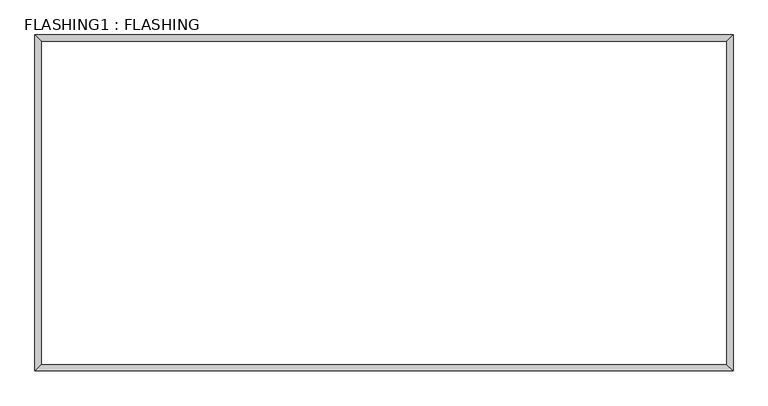
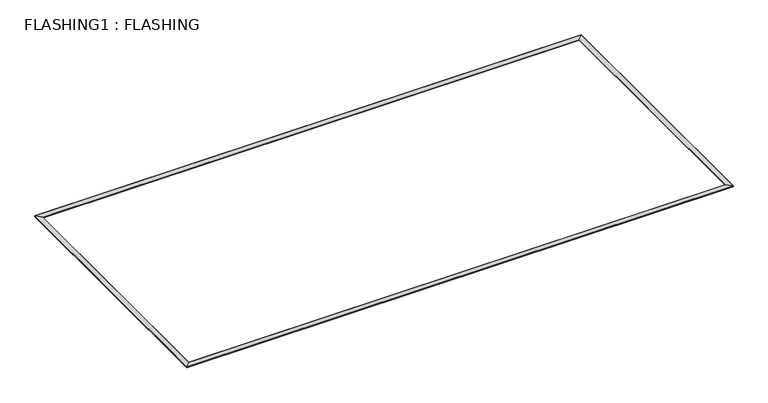
"""IFC4 building model written with IfcOpenShell, lengths in millimetres: proxy geometry, FLASHING1 : FLASHING."""

import ifcopenshell
import ifcopenshell.guid

model = None  # the IFC model being written
_history = None  # IfcOwnerHistory: only IFC2X3 demands one
_inside = {}  # id of a spatial element -> (the spatial element, [elements in it])
_under = {}  # id of a project, library or spatial element -> (it, [spatial elements below it])
_declared = {}  # id of a project -> (the project, [libraries it declares])
_typed = {}  # id of a type object -> (the type object, [elements of that type])
_made_of = {}  # id of a material, layer set ... -> (it, [elements and type objects made of it])


def new_model(schema):
    """Start an empty IFC model of exactly this schema.

    Asked for "IFC4X3", IfcOpenShell would pick the latest addendum, in which some entities
    have other attributes; the version numbers below select the first issue.
    IFC2X3 requires an IfcOwnerHistory on every rooted entity: one is made here for all.
    """
    global model, _history
    if schema == "IFC4X3":
        model = ifcopenshell.file(schema_version=(4, 3, 0, 0))
    else:
        model = ifcopenshell.file(schema=schema)
    _inside.clear()
    _under.clear()
    _declared.clear()
    _typed.clear()
    _made_of.clear()
    _history = None
    if model.schema == "IFC2X3":
        org = make("IfcOrganization", Name="unknown")
        user = make(
            "IfcPersonAndOrganization",
            ThePerson=make("IfcPerson", FamilyName="unknown"),
            TheOrganization=org,
        )
        app = make(
            "IfcApplication",
            ApplicationDeveloper=org,
            Version="unknown",
            ApplicationFullName="unknown",
            ApplicationIdentifier="unknown",
        )
        _history = make(
            "IfcOwnerHistory",
            OwningUser=user,
            OwningApplication=app,
            ChangeAction="ADDED",
            CreationDate=0,
        )
    return model


def make(cls, **values):
    """One entity of the class cls with the attributes given. An attribute that is None is left unset."""
    return model.create_entity(
        cls, **{name: value for name, value in values.items() if value is not None}
    )


def rooted(cls, **values):
    """An entity with a GlobalId (a new one), such as an element, a storey or a relation."""
    return make(cls, GlobalId=ifcopenshell.guid.new(), OwnerHistory=_history, **values)


def si_unit(unit_type, name, prefix=None):
    """IfcSIUnit, for example si_unit("LENGTHUNIT", "METRE", prefix="MILLI")."""
    return make("IfcSIUnit", UnitType=unit_type, Prefix=prefix, Name=name)


def assignment(units):
    """IfcUnitAssignment: the units of a project."""
    return None if units is None else make("IfcUnitAssignment", Units=units)


def point(xyz):
    """IfcCartesianPoint."""
    return None if xyz is None else make("IfcCartesianPoint", Coordinates=xyz)


def direction(xyz):
    """IfcDirection."""
    return None if xyz is None else make("IfcDirection", DirectionRatios=xyz)


def frame(location, z_axis=None, x_axis=None):
    """IfcAxis2Placement3D, a coordinate frame: its origin and axes. An axis left out is left unset."""
    return make(
        "IfcAxis2Placement3D",
        Location=point(location),
        Axis=direction(z_axis),
        RefDirection=direction(x_axis),
    )


def origin():
    """The frame at (0, 0, 0) with its axes left unset."""
    return frame((0.0, 0.0, 0.0))


def place(relative_to, where):
    """IfcLocalPlacement: puts the frame where relative to a parent placement (None: the world)."""
    return make(
        "IfcLocalPlacement", PlacementRelTo=relative_to, RelativePlacement=where
    )


def context(
    kind, dimensions, precision=None, world=None, true_north=None, identifier=None
):
    """IfcGeometricRepresentationContext, for example the 3D "Model" context."""
    return make(
        "IfcGeometricRepresentationContext",
        ContextIdentifier=identifier,
        ContextType=kind,
        CoordinateSpaceDimension=dimensions,
        Precision=precision,
        WorldCoordinateSystem=world,
        TrueNorth=true_north,
    )


def project(units=None, contexts=None):
    """IfcProject with its units and contexts."""
    return rooted(
        "IfcProject",
        Name="project",
        RepresentationContexts=contexts,
        UnitsInContext=assignment(units),
    )


def spatial(cls, under=None, at=None, **own):
    """A site, building, storey or space (cls), placed at a placement, below another one or the project."""
    s = rooted(cls, ObjectPlacement=at, **own)
    if under is not None:
        _under.setdefault(under.id(), (under, []))[1].append(s)
    return s


def faces_of(points, faces, orient=None, outer=None):
    """IfcFace entities. A face is a list of loops; a loop is a list of indices into points, from 0.

    orient and outer hold one flag for each loop. By default every Orientation is true, the
    first loop of a face is its IfcFaceOuterBound and the others are IfcFaceBound.
    """
    made = []
    for i, loops in enumerate(faces):
        bounds = []
        for j, loop in enumerate(loops):
            is_outer = j == 0 if outer is None else outer[i][j]
            bounds.append(
                make(
                    "IfcFaceOuterBound" if is_outer else "IfcFaceBound",
                    Bound=make("IfcPolyLoop", Polygon=[points[k] for k in loop]),
                    Orientation=True if orient is None else orient[i][j],
                )
            )
        made.append(make("IfcFace", Bounds=bounds))
    return made


def faceted_brep(points, faces, orient=None, outer=None, voids=None):
    """IfcFacetedBrep: a solid bounded by flat faces; with voids (closed shells), ...WithVoids."""
    shared = [point(p) for p in points]
    hull = make("IfcClosedShell", CfsFaces=faces_of(shared, faces, orient, outer))
    if voids is None:
        return make("IfcFacetedBrep", Outer=hull)
    return make(
        "IfcFacetedBrepWithVoids",
        Outer=hull,
        Voids=[
            make(cls, CfsFaces=faces_of(shared, fs, o, b)) for cls, fs, o, b in voids
        ],
    )


def shape(context_of_items, identifier, shape_type, items):
    """IfcShapeRepresentation: the items that make up one representation, for example the "Body"."""
    return make(
        "IfcShapeRepresentation",
        ContextOfItems=context_of_items,
        RepresentationIdentifier=identifier,
        RepresentationType=shape_type,
        Items=items,
    )


def source(mapping_origin, context_of_items, identifier, shape_type, items):
    """IfcRepresentationMap: a shape defined once, which mapped items show again and again."""
    return make(
        "IfcRepresentationMap",
        MappingOrigin=mapping_origin,
        MappedRepresentation=shape(context_of_items, identifier, shape_type, items),
    )


def transform(
    local_origin,
    x_axis=None,
    y_axis=None,
    z_axis=None,
    scale=None,
    scale2=None,
    scale3=None,
    uniform=True,
):
    """IfcCartesianTransformationOperator3D, or its non-uniform kind. x_axis, y_axis, z_axis: its Axis1, 2, 3."""
    if uniform:
        return make(
            "IfcCartesianTransformationOperator3D",
            Axis1=direction(x_axis),
            Axis2=direction(y_axis),
            LocalOrigin=point(local_origin),
            Scale=scale,
            Axis3=direction(z_axis),
        )
    return make(
        "IfcCartesianTransformationOperator3DnonUniform",
        Axis1=direction(x_axis),
        Axis2=direction(y_axis),
        LocalOrigin=point(local_origin),
        Scale=scale,
        Axis3=direction(z_axis),
        Scale2=scale2,
        Scale3=scale3,
    )


def mapped(mapping_source, mapping_target):
    """IfcMappedItem: shows the shape of a source again, moved by a transform."""
    return make(
        "IfcMappedItem", MappingSource=mapping_source, MappingTarget=mapping_target
    )


def made_of(thing, what):
    """Note that an element or type object is made of a material, layer set ...; save() writes the relation."""
    if what is not None:
        _made_of.setdefault(what.id(), (what, []))[1].append(thing)
    return thing


def element(
    cls,
    number,
    at=None,
    inside=None,
    cuts=None,
    type_object=None,
    material=None,
    context=None,
    identifier="Body",
    shape_type=None,
    held_by="IfcProductDefinitionShape",
    body=None,
    shapes=None,
    **own,
):
    """One element of the class cls, such as IfcWall. Its Tag is "e" and its number.

    at: its placement. inside: the storey or other place that contains it. cuts: it is an
    opening in that element (IfcRelVoidsElement). A single representation is given by context,
    identifier, shape_type and body (its items); several are given by shapes. held_by: the class
    of the entity that holds the representations. save() writes the other relations.
    """
    e = rooted(cls, Tag="e%d" % number, ObjectPlacement=at, **own)
    if body is not None:
        shapes = [shape(context, identifier, shape_type, body)]
    if shapes is not None:
        e.Representation = make(held_by, Representations=shapes)
    if inside is not None:
        _inside.setdefault(inside.id(), (inside, []))[1].append(e)
    if cuts is not None:
        rooted(
            "IfcRelVoidsElement", RelatingBuildingElement=cuts, RelatedOpeningElement=e
        )
    if type_object is not None:
        _typed.setdefault(type_object.id(), (type_object, []))[1].append(e)
    return made_of(e, material)


def aggregate(whole, parts):
    """IfcRelAggregates: a whole, such as a stair, and the parts it consists of."""
    return rooted("IfcRelAggregates", RelatingObject=whole, RelatedObjects=parts)


def save(model, path):
    """Write the relations noted so far, then the file.

    IfcRelAggregates (storeys below a building ...), IfcRelContainedInSpatialStructure (elements
    in a storey), IfcRelDefinesByType, IfcRelAssociatesMaterial and IfcRelDeclares: one each for
    every whole, place, type object, material and project.
    """
    for whole, parts in _under.values():
        aggregate(whole, parts)
    for where, things in _inside.values():
        rooted(
            "IfcRelContainedInSpatialStructure",
            RelatedElements=things,
            RelatingStructure=where,
        )
    for kind, things in _typed.values():
        rooted("IfcRelDefinesByType", RelatedObjects=things, RelatingType=kind)
    for what, things in _made_of.values():
        rooted("IfcRelAssociatesMaterial", RelatedObjects=things, RelatingMaterial=what)
    for by, libraries in _declared.values():
        rooted("IfcRelDeclares", RelatingContext=by, RelatedDefinitions=libraries)
    model.write(path)


def flashing1_flashing_4cce81cf(model_context):
    return source(origin(), model_context, "Body", "Brep", [
        faceted_brep([(40720.0, 40009.5208589, 18739.9720055), (40720.0, 40009.5208589, 18724.9720055), (40720.0, 19989.5208589, 18724.9720055), (40720.0, 19989.5208589, 18739.9720055), (40721.0, 40010.5208589, 18750.9720055), (40721.0, 40010.5208589, 18739.9720055), (40721.0, 19988.5208589, 18739.9720055), (40721.0, 19988.5208589, 18750.9720055), (40749.0, 40038.5208589, 18819.1280996), (40749.0, 40038.5208589, 18750.9720055), (40749.0, 19960.5208589, 18750.9720055), (40749.0, 19960.5208589, 18819.1280996), (40371.0, 39660.5208589, 18804.3045702), (40371.0, 20338.5208589, 18804.3045702), (40371.0, 39660.5208589, 18750.9720055), (40371.0, 20338.5208589, 18750.9720055), (40399.0, 39688.5208589, 18739.9720055), (40399.0, 39688.5208589, 18750.9720055), (40399.0, 20310.5208589, 18750.9720055), (40399.0, 20310.5208589, 18739.9720055), (40400.0, 39689.5208589, 18724.9720055), (40400.0, 39689.5208589, 18739.9720055), (40400.0, 20309.5208589, 18739.9720055), (40400.0, 20309.5208589, 18724.9720055), (40398.0, 39687.5208589, 18749.9720055), (40398.0, 39687.5208589, 18724.9720055), (40398.0, 20311.5208589, 18724.9720055), (40398.0, 20311.5208589, 18749.9720055), (40370.0, 39659.5208589, 18805.2661232), (40370.0, 39659.5208589, 18749.9720055), (40370.0, 20339.5208589, 18749.9720055), (40370.0, 20339.5208589, 18805.2661232), (40750.0, 40039.5208589, 18820.168084), (40750.0, 19959.5208589, 18820.168084), (40750.0, 40039.5208589, 18749.9720055), (40750.0, 19959.5208589, 18749.9720055), (40722.0, 40011.5208589, 18724.9720055), (40722.0, 40011.5208589, 18749.9720055), (40722.0, 19987.5208589, 18749.9720055), (40722.0, 19987.5208589, 18724.9720055), (-935.0, 19989.5208589, 18724.9720055), (-935.0, 19989.5208589, 18739.9720055), (-936.0, 19988.5208589, 18739.9720055), (-936.0, 19988.5208589, 18750.9720055), (-964.0, 19960.5208589, 18750.9720055), (-964.0, 19960.5208589, 18819.1280996), (-586.0, 20338.5208589, 18804.3045702), (-586.0, 20338.5208589, 18750.9720055), (-614.0, 20310.5208589, 18750.9720055), (-614.0, 20310.5208589, 18739.9720055), (-615.0, 20309.5208589, 18739.9720055), (-615.0, 20309.5208589, 18724.9720055), (-613.0, 20311.5208589, 18724.9720055), (-613.0, 20311.5208589, 18749.9720055), (-585.0, 20339.5208589, 18749.9720055), (-585.0, 20339.5208589, 18805.2661232), (-965.0, 19959.5208589, 18820.168084), (-965.0, 19959.5208589, 18749.9720055), (-937.0, 19987.5208589, 18749.9720055), (-937.0, 19987.5208589, 18724.9720055), (-935.0, 40009.5208589, 18724.9720055), (-935.0, 40009.5208589, 18739.9720055), (-936.0, 40010.5208589, 18739.9720055), (-936.0, 40010.5208589, 18750.9720055), (-964.0, 40038.5208589, 18750.9720055), (-964.0, 40038.5208589, 18819.1280996), (-586.0, 39660.5208589, 18804.3045702), (-586.0, 39660.5208589, 18750.9720055), (-614.0, 39688.5208589, 18750.9720055), (-614.0, 39688.5208589, 18739.9720055), (-615.0, 39689.5208589, 18739.9720055), (-615.0, 39689.5208589, 18724.9720055), (-613.0, 39687.5208589, 18724.9720055), (-613.0, 39687.5208589, 18749.9720055), (-585.0, 39659.5208589, 18749.9720055), (-585.0, 39659.5208589, 18805.2661232), (-965.0, 40039.5208589, 18820.168084), (-965.0, 40039.5208589, 18749.9720055), (-937.0, 40011.5208589, 18749.9720055), (-937.0, 40011.5208589, 18724.9720055)], [[[0, 1, 2, 3]], [[4, 5, 6, 7]], [[8, 9, 10, 11]], [[12, 8, 11, 13]], [[14, 12, 13, 15]], [[16, 17, 18, 19]], [[20, 21, 22, 23]], [[24, 25, 26, 27]], [[28, 29, 30, 31]], [[32, 28, 31, 33]], [[34, 32, 33, 35]], [[36, 37, 38, 39]], [[3, 2, 40, 41]], [[7, 6, 42, 43]], [[11, 10, 44, 45]], [[13, 11, 45, 46]], [[15, 13, 46, 47]], [[19, 18, 48, 49]], [[23, 22, 50, 51]], [[27, 26, 52, 53]], [[31, 30, 54, 55]], [[33, 31, 55, 56]], [[35, 33, 56, 57]], [[39, 38, 58, 59]], [[41, 40, 60, 61]], [[43, 42, 62, 63]], [[45, 44, 64, 65]], [[46, 45, 65, 66]], [[47, 46, 66, 67]], [[49, 48, 68, 69]], [[51, 50, 70, 71]], [[53, 52, 72, 73]], [[55, 54, 74, 75]], [[56, 55, 75, 76]], [[57, 56, 76, 77]], [[59, 58, 78, 79]], [[61, 60, 1, 0]], [[5, 62, 42, 6], [3, 41, 61, 0]], [[63, 62, 5, 4]], [[9, 64, 44, 10], [7, 43, 63, 4]], [[65, 64, 9, 8]], [[66, 65, 8, 12]], [[67, 66, 12, 14]], [[17, 68, 48, 18], [15, 47, 67, 14]], [[69, 68, 17, 16]], [[21, 70, 50, 22], [19, 49, 69, 16]], [[71, 70, 21, 20]], [[23, 51, 71, 20], [25, 72, 52, 26]], [[73, 72, 25, 24]], [[27, 53, 73, 24], [29, 74, 54, 30]], [[75, 74, 29, 28]], [[76, 75, 28, 32]], [[77, 76, 32, 34]], [[35, 57, 77, 34], [37, 78, 58, 38]], [[79, 78, 37, 36]], [[39, 59, 79, 36], [1, 60, 40, 2]]]),
    ])


if __name__ == "__main__":
    model = new_model("IFC4")
    model_context = context("Model", 3, world=origin())
    ifc_project = project(units=[si_unit("LENGTHUNIT", "METRE", prefix="MILLI")], contexts=[model_context])
    site = spatial("IfcSite", under=ifc_project)
    building = spatial("IfcBuilding", under=site)
    placement = place(None, origin())
    flashing1_flashing_shape = flashing1_flashing_4cce81cf(model_context)
    element("IfcBuildingElementProxy", 1, Name="FLASHING1 : FLASHING", ObjectType="FLASHING1 : FLASHING", at=placement, inside=building, context=model_context, shape_type="MappedRepresentation", body=[
        mapped(flashing1_flashing_shape, transform((0.0, 0.0, 0.0), x_axis=(1.0, 0.0, 0.0), y_axis=(0.0, 1.0, 0.0), z_axis=(0.0, 0.0, 1.0))),
    ])
    save(model, "model.ifc")
